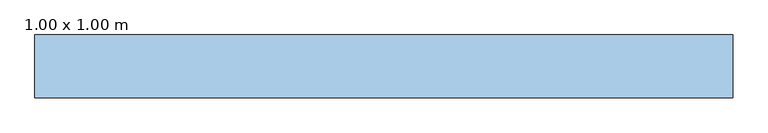
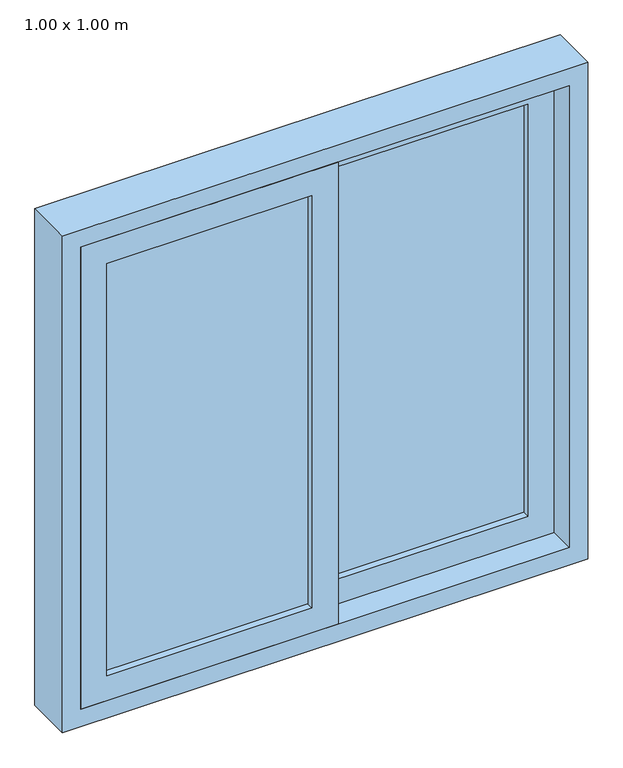
"""IFC4 building model written with IfcOpenShell, lengths in millimetres: window geometry, Janela de correr vidro - 2 Folhas : 1.00 x 1.00 m."""

from ifc_helpers import new_model, si_unit, frame, origin, place, context, project, spatial, polyline, outline, extrude, source, transform, mapped, element, save


def window_1_00_x_1_00_m_107850cb(model_context):
    return source(origin(), model_context, "Body", "SweptSolid", [
        extrude(outline(polyline([(935.0, -25.0), (935.0, 465.0), (1865.0, 465.0), (1865.0, -25.0), (935.0, -25.0)]), holes=[polyline([(1815.0, 25.0), (1815.0, 415.0), (985.0, 415.0), (985.0, 25.0), (1815.0, 25.0)])]), frame((0.0, -25.0, 0.0), z_axis=(0.0, 1.0, 0.0), x_axis=(0.0, 0.0, 1.0)), (0.0, 0.0, 1.0), 40.0),
        extrude(outline(polyline([(1865.0, 25.0), (1865.0, -465.0), (935.0, -465.0), (935.0, 25.0), (1865.0, 25.0)]), holes=[polyline([(985.0, -25.0), (985.0, -415.0), (1815.0, -415.0), (1815.0, -25.0), (985.0, -25.0)])]), frame((0.0, -75.0, 0.0), z_axis=(0.0, 1.0, 0.0), x_axis=(0.0, 0.0, 1.0)), (0.0, 0.0, 1.0), 40.0),
        extrude(outline(polyline([(1900.0, 500.0), (1900.0, -500.0), (900.0, -500.0), (900.0, 500.0), (1900.0, 500.0)]), holes=[polyline([(935.0, 465.0), (935.0, -465.0), (1865.0, -465.0), (1865.0, 465.0), (935.0, 465.0)])]), frame((0.0, -75.0, 0.0), z_axis=(0.0, 1.0, 0.0), x_axis=(0.0, 0.0, 1.0)), (0.0, 0.0, 1.0), 90.0),
        extrude(outline(polyline([(25.0, 2.0), (415.0, 2.0), (415.0, -12.0), (25.0, -12.0), (25.0, 2.0)])), frame((0.0, 0.0, 985.0), z_axis=(0.0, 0.0, 1.0), x_axis=(1.0, 0.0, 0.0)), (0.0, 0.0, 1.0), 830.0),
        extrude(outline(polyline([(-415.0, -48.0), (-25.0, -48.0), (-25.0, -62.0), (-415.0, -62.0), (-415.0, -48.0)])), frame((0.0, 0.0, 985.0), z_axis=(0.0, 0.0, 1.0), x_axis=(1.0, 0.0, 0.0)), (0.0, 0.0, 1.0), 830.0),
    ])


if __name__ == "__main__":
    model = new_model("IFC4")
    model_context = context("Model", 3, world=origin())
    ifc_project = project(units=[si_unit("LENGTHUNIT", "METRE", prefix="MILLI")], contexts=[model_context])
    site = spatial("IfcSite", under=ifc_project)
    building = spatial("IfcBuilding", under=site)
    placement = place(None, origin())
    window_1_00_x_1_00_m_shape = window_1_00_x_1_00_m_107850cb(model_context)
    element("IfcWindow", 1, ObjectType="Janela de correr vidro - 2 Folhas : 1.00 x 1.00 m", at=placement, inside=building, context=model_context, shape_type="MappedRepresentation", body=[
        mapped(window_1_00_x_1_00_m_shape, transform((0.0, 0.0, 0.0), x_axis=(1.0, 0.0, 0.0), y_axis=(0.0, 1.0, 0.0), z_axis=(0.0, 0.0, 1.0))),
    ])
    save(model, "model.ifc")

# Revit data of these elements
# Type "Janela de correr vidro - 2 Folhas : 1.00 x 1.00 m"
#   Type Mark = "J26"
#   Construction Type Id = "GSP4R"
#   Analytic Construction = "Vidraça única Pilkington 1/8 pol"
#   Visual Light Transmittance = 0.9
#   Thermal Resistance (R) = 0.271106 (m²·K)/W
#   Solar Heat Gain Coefficient = 0.78
#   Rough Width = 1.000 m
#   Rough Height = 1.000 m
#   Largura da moldura do painel = 0.050 m
#   Espessura da moldura do painel = 0.040 m
#   Height = 1.000 m
#   Heat Transfer Coefficient (U) = 3.6886 W/(m²·K)
#   Largura da estrutura = 0.035 m
#   Espessura da moldura = 0.090 m
#   Altura-padrão do peitoril = 0.900 m
#   Width = 1.000 m
#   Pingadeira = yes
#   Material da Pingadeira = Granito amarelo
#   Vidro = Vidro
#   Material da estrutura = Metal - Alumínio
#   Wall Closure = (empty or 0)
# Element 1 (IfcWindow, "Janela de correr vidro - 2 Folhas : 1.00 x 1.00 m")
#   Materials on its faces: "Metal - Alumínio", "Vidro"
# Materials
#   "Granito amarelo": class "Genérico", colour RGB 80 80 80, transparency 0, Cost = 0
#   "Vidro": class "Vidro", colour RGB 0 128 192, transparency 0.9
#   "Metal - Alumínio": class "Metal", colour RGB 247 247 247, transparency 0
